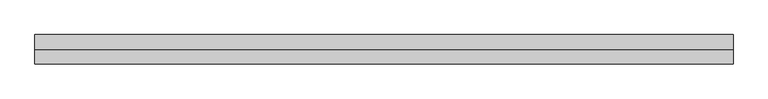
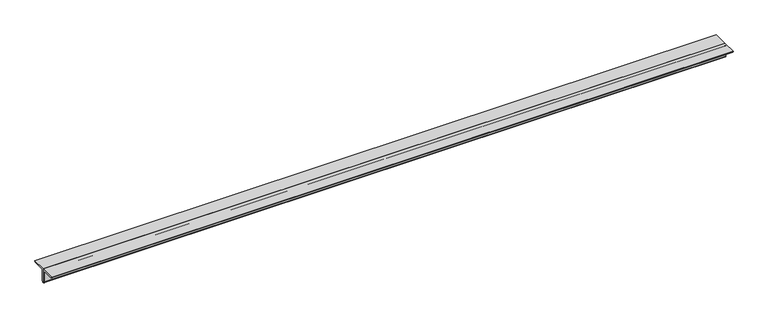
"""IFC4 building model written with IfcOpenShell, lengths in millimetres: member geometry, Steel Framing_2Ls_KS : H_SB_AR_S02_2Ls-100x100x10_VBR1."""

import ifcopenshell
import ifcopenshell.guid

model = None  # the IFC model being written
_history = None  # IfcOwnerHistory: only IFC2X3 demands one
_inside = {}  # id of a spatial element -> (the spatial element, [elements in it])
_under = {}  # id of a project, library or spatial element -> (it, [spatial elements below it])
_declared = {}  # id of a project -> (the project, [libraries it declares])
_typed = {}  # id of a type object -> (the type object, [elements of that type])
_made_of = {}  # id of a material, layer set ... -> (it, [elements and type objects made of it])


def new_model(schema):
    """Start an empty IFC model of exactly this schema.

    Asked for "IFC4X3", IfcOpenShell would pick the latest addendum, in which some entities
    have other attributes; the version numbers below select the first issue.
    IFC2X3 requires an IfcOwnerHistory on every rooted entity: one is made here for all.
    """
    global model, _history
    if schema == "IFC4X3":
        model = ifcopenshell.file(schema_version=(4, 3, 0, 0))
    else:
        model = ifcopenshell.file(schema=schema)
    _inside.clear()
    _under.clear()
    _declared.clear()
    _typed.clear()
    _made_of.clear()
    _history = None
    if model.schema == "IFC2X3":
        org = make("IfcOrganization", Name="unknown")
        user = make(
            "IfcPersonAndOrganization",
            ThePerson=make("IfcPerson", FamilyName="unknown"),
            TheOrganization=org,
        )
        app = make(
            "IfcApplication",
            ApplicationDeveloper=org,
            Version="unknown",
            ApplicationFullName="unknown",
            ApplicationIdentifier="unknown",
        )
        _history = make(
            "IfcOwnerHistory",
            OwningUser=user,
            OwningApplication=app,
            ChangeAction="ADDED",
            CreationDate=0,
        )
    return model


def make(cls, **values):
    """One entity of the class cls with the attributes given. An attribute that is None is left unset."""
    return model.create_entity(
        cls, **{name: value for name, value in values.items() if value is not None}
    )


def rooted(cls, **values):
    """An entity with a GlobalId (a new one), such as an element, a storey or a relation."""
    return make(cls, GlobalId=ifcopenshell.guid.new(), OwnerHistory=_history, **values)


def si_unit(unit_type, name, prefix=None):
    """IfcSIUnit, for example si_unit("LENGTHUNIT", "METRE", prefix="MILLI")."""
    return make("IfcSIUnit", UnitType=unit_type, Prefix=prefix, Name=name)


def assignment(units):
    """IfcUnitAssignment: the units of a project."""
    return None if units is None else make("IfcUnitAssignment", Units=units)


def point(xyz):
    """IfcCartesianPoint."""
    return None if xyz is None else make("IfcCartesianPoint", Coordinates=xyz)


def direction(xyz):
    """IfcDirection."""
    return None if xyz is None else make("IfcDirection", DirectionRatios=xyz)


def frame(location, z_axis=None, x_axis=None):
    """IfcAxis2Placement3D, a coordinate frame: its origin and axes. An axis left out is left unset."""
    return make(
        "IfcAxis2Placement3D",
        Location=point(location),
        Axis=direction(z_axis),
        RefDirection=direction(x_axis),
    )


def frame_2d(location, x_axis=None):
    """IfcAxis2Placement2D, a coordinate frame in the plane: its origin and x axis."""
    return make(
        "IfcAxis2Placement2D", Location=point(location), RefDirection=direction(x_axis)
    )


def origin():
    """The frame at (0, 0, 0) with its axes left unset."""
    return frame((0.0, 0.0, 0.0))


def place(relative_to, where):
    """IfcLocalPlacement: puts the frame where relative to a parent placement (None: the world)."""
    return make(
        "IfcLocalPlacement", PlacementRelTo=relative_to, RelativePlacement=where
    )


def context(
    kind, dimensions, precision=None, world=None, true_north=None, identifier=None
):
    """IfcGeometricRepresentationContext, for example the 3D "Model" context."""
    return make(
        "IfcGeometricRepresentationContext",
        ContextIdentifier=identifier,
        ContextType=kind,
        CoordinateSpaceDimension=dimensions,
        Precision=precision,
        WorldCoordinateSystem=world,
        TrueNorth=true_north,
    )


def project(units=None, contexts=None):
    """IfcProject with its units and contexts."""
    return rooted(
        "IfcProject",
        Name="project",
        RepresentationContexts=contexts,
        UnitsInContext=assignment(units),
    )


def spatial(cls, under=None, at=None, **own):
    """A site, building, storey or space (cls), placed at a placement, below another one or the project."""
    s = rooted(cls, ObjectPlacement=at, **own)
    if under is not None:
        _under.setdefault(under.id(), (under, []))[1].append(s)
    return s


def polyline(points):
    """IfcPolyline through the points."""
    return make("IfcPolyline", Points=[point(p) for p in points])


def circle_curve(where, radius):
    """IfcCircle in the frame where."""
    return make("IfcCircle", Position=where, Radius=radius)


def trimmed(basis, trim1, trim2, sense, master):
    """IfcTrimmedCurve: the piece of a basis curve between two trims."""
    return make(
        "IfcTrimmedCurve",
        BasisCurve=basis,
        Trim1=trim1,
        Trim2=trim2,
        SenseAgreement=sense,
        MasterRepresentation=master,
    )


def segment(curve, same_sense, transition):
    """IfcCompositeCurveSegment."""
    return make(
        "IfcCompositeCurveSegment",
        Transition=transition,
        SameSense=same_sense,
        ParentCurve=curve,
    )


def composite_curve(segments, self_intersect=None):
    """IfcCompositeCurve: segments joined end to end."""
    return make("IfcCompositeCurve", Segments=segments, SelfIntersect=self_intersect)


def outline(outer, holes=None, kind="AREA"):
    """IfcArbitraryClosedProfileDef: a profile drawn as a closed curve; with holes, ...WithVoids."""
    if holes is None:
        return make("IfcArbitraryClosedProfileDef", ProfileType=kind, OuterCurve=outer)
    return make(
        "IfcArbitraryProfileDefWithVoids",
        ProfileType=kind,
        OuterCurve=outer,
        InnerCurves=holes,
    )


def extrude(swept, where, along, depth):
    """IfcExtrudedAreaSolid: the profile swept, set in the frame where, extruded along a direction by depth."""
    return make(
        "IfcExtrudedAreaSolid",
        SweptArea=swept,
        Position=where,
        ExtrudedDirection=direction(along),
        Depth=depth,
    )


def shape(context_of_items, identifier, shape_type, items):
    """IfcShapeRepresentation: the items that make up one representation, for example the "Body"."""
    return make(
        "IfcShapeRepresentation",
        ContextOfItems=context_of_items,
        RepresentationIdentifier=identifier,
        RepresentationType=shape_type,
        Items=items,
    )


def source(mapping_origin, context_of_items, identifier, shape_type, items):
    """IfcRepresentationMap: a shape defined once, which mapped items show again and again."""
    return make(
        "IfcRepresentationMap",
        MappingOrigin=mapping_origin,
        MappedRepresentation=shape(context_of_items, identifier, shape_type, items),
    )


def transform(
    local_origin,
    x_axis=None,
    y_axis=None,
    z_axis=None,
    scale=None,
    scale2=None,
    scale3=None,
    uniform=True,
):
    """IfcCartesianTransformationOperator3D, or its non-uniform kind. x_axis, y_axis, z_axis: its Axis1, 2, 3."""
    if uniform:
        return make(
            "IfcCartesianTransformationOperator3D",
            Axis1=direction(x_axis),
            Axis2=direction(y_axis),
            LocalOrigin=point(local_origin),
            Scale=scale,
            Axis3=direction(z_axis),
        )
    return make(
        "IfcCartesianTransformationOperator3DnonUniform",
        Axis1=direction(x_axis),
        Axis2=direction(y_axis),
        LocalOrigin=point(local_origin),
        Scale=scale,
        Axis3=direction(z_axis),
        Scale2=scale2,
        Scale3=scale3,
    )


def mapped(mapping_source, mapping_target):
    """IfcMappedItem: shows the shape of a source again, moved by a transform."""
    return make(
        "IfcMappedItem", MappingSource=mapping_source, MappingTarget=mapping_target
    )


def made_of(thing, what):
    """Note that an element or type object is made of a material, layer set ...; save() writes the relation."""
    if what is not None:
        _made_of.setdefault(what.id(), (what, []))[1].append(thing)
    return thing


def element(
    cls,
    number,
    at=None,
    inside=None,
    cuts=None,
    type_object=None,
    material=None,
    context=None,
    identifier="Body",
    shape_type=None,
    held_by="IfcProductDefinitionShape",
    body=None,
    shapes=None,
    **own,
):
    """One element of the class cls, such as IfcWall. Its Tag is "e" and its number.

    at: its placement. inside: the storey or other place that contains it. cuts: it is an
    opening in that element (IfcRelVoidsElement). A single representation is given by context,
    identifier, shape_type and body (its items); several are given by shapes. held_by: the class
    of the entity that holds the representations. save() writes the other relations.
    """
    e = rooted(cls, Tag="e%d" % number, ObjectPlacement=at, **own)
    if body is not None:
        shapes = [shape(context, identifier, shape_type, body)]
    if shapes is not None:
        e.Representation = make(held_by, Representations=shapes)
    if inside is not None:
        _inside.setdefault(inside.id(), (inside, []))[1].append(e)
    if cuts is not None:
        rooted(
            "IfcRelVoidsElement", RelatingBuildingElement=cuts, RelatedOpeningElement=e
        )
    if type_object is not None:
        _typed.setdefault(type_object.id(), (type_object, []))[1].append(e)
    return made_of(e, material)


def aggregate(whole, parts):
    """IfcRelAggregates: a whole, such as a stair, and the parts it consists of."""
    return rooted("IfcRelAggregates", RelatingObject=whole, RelatedObjects=parts)


def save(model, path):
    """Write the relations noted so far, then the file.

    IfcRelAggregates (storeys below a building ...), IfcRelContainedInSpatialStructure (elements
    in a storey), IfcRelDefinesByType, IfcRelAssociatesMaterial and IfcRelDeclares: one each for
    every whole, place, type object, material and project.
    """
    for whole, parts in _under.values():
        aggregate(whole, parts)
    for where, things in _inside.values():
        rooted(
            "IfcRelContainedInSpatialStructure",
            RelatedElements=things,
            RelatingStructure=where,
        )
    for kind, things in _typed.values():
        rooted("IfcRelDefinesByType", RelatedObjects=things, RelatingType=kind)
    for what, things in _made_of.values():
        rooted("IfcRelAssociatesMaterial", RelatedObjects=things, RelatingMaterial=what)
    for by, libraries in _declared.values():
        rooted("IfcRelDeclares", RelatingContext=by, RelatedDefinitions=libraries)
    model.write(path)


def member_9746b210(model_context):
    return source(origin(), model_context, "Body", "SweptSolid", [
        extrude(outline(composite_curve([segment(polyline([(0.0, 28.2), (100.0, 28.2)]), True, "CONTINUOUS"), segment(trimmed(circle_curve(frame_2d((90.0, 28.2)), 10.0), [point((100.0, 28.2))], [point((90.0, 18.2))], False, "CARTESIAN"), True, "CONTINUOUS"), segment(polyline([(90.0, 18.2), (20.0, 18.2)]), True, "CONTINUOUS"), segment(trimmed(circle_curve(frame_2d((20.0, 8.2)), 10.0), [point((20.0, 18.2))], [point((10.0, 8.2))], True, "CARTESIAN"), True, "CONTINUOUS"), segment(polyline([(10.0, 8.2), (10.0, -61.8)]), True, "CONTINUOUS"), segment(trimmed(circle_curve(frame_2d((0.0, -61.8)), 10.0), [point((10.0, -61.8))], [point((0.0, -71.8))], False, "CARTESIAN"), True, "CONTINUOUS"), segment(polyline([(0.0, -71.8), (0.0, 28.2)]), True, "CONTINUOUS")], self_intersect=False)), frame((-2072.1213123, 0.0, 0.0), z_axis=(1.0, 0.0, 0.0), x_axis=(0.0, 1.0, 0.0)), (0.0, 0.0, 1.0), 4738.656697),
        extrude(outline(composite_curve([segment(polyline([(0.0, 28.2), (0.0, -71.8)]), True, "CONTINUOUS"), segment(trimmed(circle_curve(frame_2d((0.0, -61.8)), 10.0), [point((0.0, -71.8))], [point((-10.0, -61.8))], False, "CARTESIAN"), True, "CONTINUOUS"), segment(polyline([(-10.0, -61.8), (-10.0, 8.2)]), True, "CONTINUOUS"), segment(trimmed(circle_curve(frame_2d((-20.0, 8.2)), 10.0), [point((-10.0, 8.2))], [point((-20.0, 18.2))], True, "CARTESIAN"), True, "CONTINUOUS"), segment(polyline([(-20.0, 18.2), (-90.0, 18.2)]), True, "CONTINUOUS"), segment(trimmed(circle_curve(frame_2d((-90.0, 28.2)), 10.0), [point((-90.0, 18.2))], [point((-100.0, 28.2))], False, "CARTESIAN"), True, "CONTINUOUS"), segment(polyline([(-100.0, 28.2), (0.0, 28.2)]), True, "CONTINUOUS")], self_intersect=False)), frame((-2072.1213123, 0.0, 0.0), z_axis=(1.0, 0.0, 0.0), x_axis=(0.0, 1.0, 0.0)), (0.0, 0.0, 1.0), 4738.656697),
    ])


if __name__ == "__main__":
    model = new_model("IFC4")
    model_context = context("Model", 3, world=origin())
    ifc_project = project(units=[si_unit("LENGTHUNIT", "METRE", prefix="MILLI")], contexts=[model_context])
    site = spatial("IfcSite", under=ifc_project)
    building = spatial("IfcBuilding", under=site)
    placement = place(None, origin())
    member_shape = member_9746b210(model_context)
    element("IfcMember", 1, ObjectType="Steel Framing_2Ls_KS : H_SB_AR_S02_2Ls-100x100x10_VBR1", at=placement, inside=building, context=model_context, shape_type="MappedRepresentation", body=[
        mapped(member_shape, transform((0.0, 0.0, 0.0), x_axis=(1.0, 0.0, 0.0), y_axis=(0.0, 1.0, 0.0), z_axis=(0.0, 0.0, 1.0))),
    ])
    save(model, "model.ifc")

# Revit data of these elements
# Type "Steel Framing_2Ls_KS : H_SB_AR_S02_2Ls-100x100x10_VBR1"
#   Type Comments = "MAIN"
#   Type Mark = "VBR1"
#   H_SectionID = "2Ls-100x100x10"
#   Assembly Code = "B10"
#   Legs = "LLBB"
#   H_Ratio for Additional Steel Plate = 0.2
#   W = 0
#   Perimeter = 0.80 m²/m
#   Nominal Weight = 29.80 kgf/m
#   Length [instance default] = 1524 mm
#   Space = 0 mm
#   b = 100 mm
#   d = 100 mm
#   t = 10 mm
#   y = 28.2 mm
#   A = 0.0038 m²
#   Structural Material [instance default] = Steel, 45-345
# Element 1 (IfcMember, "Steel Framing_2Ls_KS : H_SB_AR_S02_2Ls-100x100x10_VBR1")
#   Materials on its faces: "Steel, 45-345"
# Materials
#   "Steel, 45-345": class "Metal", colour RGB 189 187 185, transparency 0, Description = "Steel 345 MPa", Cost = 0
